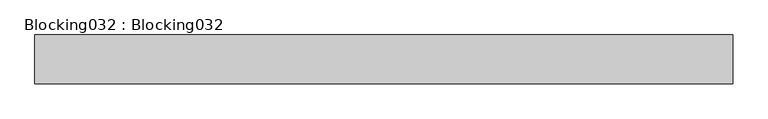
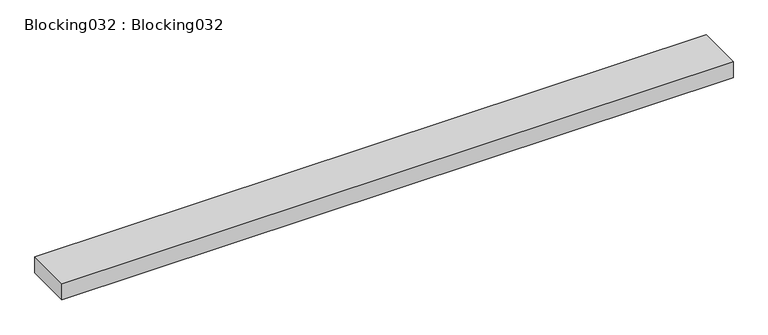
"""IFC4 building model written with IfcOpenShell, lengths in millimetres: proxy geometry, Blocking032 : Blocking032."""

from ifc_helpers import new_model, si_unit, frame, origin, place, context, project, spatial, polyline, outline, extrude, source, transform, mapped, element, save


def blocking032_blocking032_cbfbee9c(model_context):
    return source(origin(), model_context, "Body", "SweptSolid", [
        extrude(outline(polyline([(14383.0178845, -4497.8425368), (14383.0178845, -4637.5425368), (12383.0178845, -4637.5425368), (12383.0178845, -4497.8425368), (14383.0178845, -4497.8425368)])), frame((0.0, 0.0, 39655.496), z_axis=(0.0, 0.0, 1.0), x_axis=(1.0, 0.0, 0.0)), (0.0, 0.0, 1.0), 50.8),
    ])


if __name__ == "__main__":
    model = new_model("IFC4")
    model_context = context("Model", 3, world=origin())
    ifc_project = project(units=[si_unit("LENGTHUNIT", "METRE", prefix="MILLI")], contexts=[model_context])
    site = spatial("IfcSite", under=ifc_project)
    building = spatial("IfcBuilding", under=site)
    placement = place(None, origin())
    blocking032_blocking032_shape = blocking032_blocking032_cbfbee9c(model_context)
    element("IfcBuildingElementProxy", 1, Name="Blocking032 : Blocking032", ObjectType="Blocking032 : Blocking032", at=placement, inside=building, context=model_context, shape_type="MappedRepresentation", body=[
        mapped(blocking032_blocking032_shape, transform((0.0, 0.0, 0.0), x_axis=(1.0, 0.0, 0.0), y_axis=(0.0, 1.0, 0.0), z_axis=(0.0, 0.0, 1.0))),
    ])
    save(model, "model.ifc")

# Revit data of these elements
# Type "Blocking032 : Blocking032"
#   NameOverride = "Blocking032"
# Element 1 (IfcBuildingElementProxy, "Blocking032 : Blocking032")
#   Materials on its faces: "WOOD BLOCKING AS REQUIRED"
# Materials
#   "WOOD BLOCKING AS REQUIRED": class "Unassigned", colour RGB 166 124 85, transparency 0, Cost = 0
